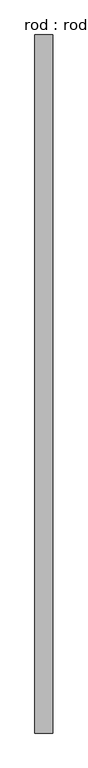
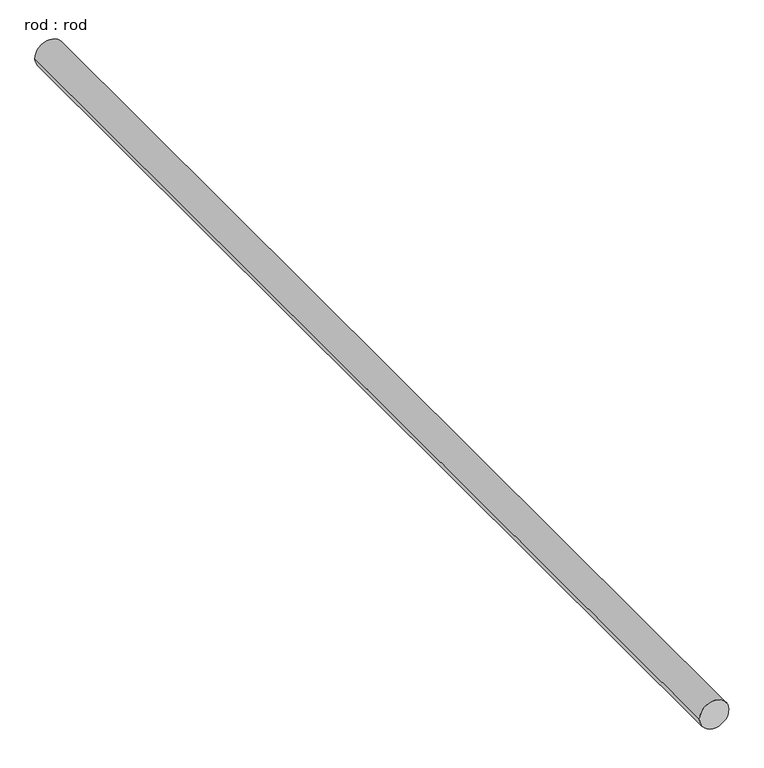
"""IFC4 building model written with IfcOpenShell, lengths in millimetres: proxy geometry, rod : rod."""

from ifc_helpers import new_model, si_unit, point, frame, frame_2d, origin, place, context, project, spatial, circle_curve, trimmed, segment, composite_curve, outline, extrude, source, transform, mapped, element, save


def rod_rod_bedfcf5f(model_context):
    return source(origin(), model_context, "Body", "SweptSolid", [
        extrude(outline(composite_curve([segment(trimmed(circle_curve(frame_2d((0.0108462, 0.0)), 200.0), [point((0.0108462, 200.0))], [point((0.0108462, -200.0))], False, "CARTESIAN"), True, "CONTINUOUS"), segment(trimmed(circle_curve(frame_2d((0.0108462, 0.0)), 200.0), [point((0.0108462, -200.0))], [point((0.0108462, 200.0))], False, "CARTESIAN"), True, "CONTINUOUS")], self_intersect=False)), frame((0.0, -3754.4621417, 0.0), z_axis=(0.0, 1.0, 0.0), x_axis=(0.0, 0.0, 1.0)), (0.0, 0.0, 1.0), 15694.3815141),
    ])


if __name__ == "__main__":
    model = new_model("IFC4")
    model_context = context("Model", 3, world=origin())
    ifc_project = project(units=[si_unit("LENGTHUNIT", "METRE", prefix="MILLI")], contexts=[model_context])
    site = spatial("IfcSite", under=ifc_project)
    building = spatial("IfcBuilding", under=site)
    placement = place(None, origin())
    rod_rod_shape = rod_rod_bedfcf5f(model_context)
    element("IfcBuildingElementProxy", 1, Name="rod : rod", ObjectType="rod : rod", at=placement, inside=building, context=model_context, shape_type="MappedRepresentation", body=[
        mapped(rod_rod_shape, transform((0.0, 0.0, 0.0), x_axis=(1.0, 0.0, 0.0), y_axis=(0.0, 1.0, 0.0), z_axis=(0.0, 0.0, 1.0))),
    ])
    save(model, "model.ifc")

# Revit data of these elements
# Type "rod : rod"
#   Default Elevation = 0
